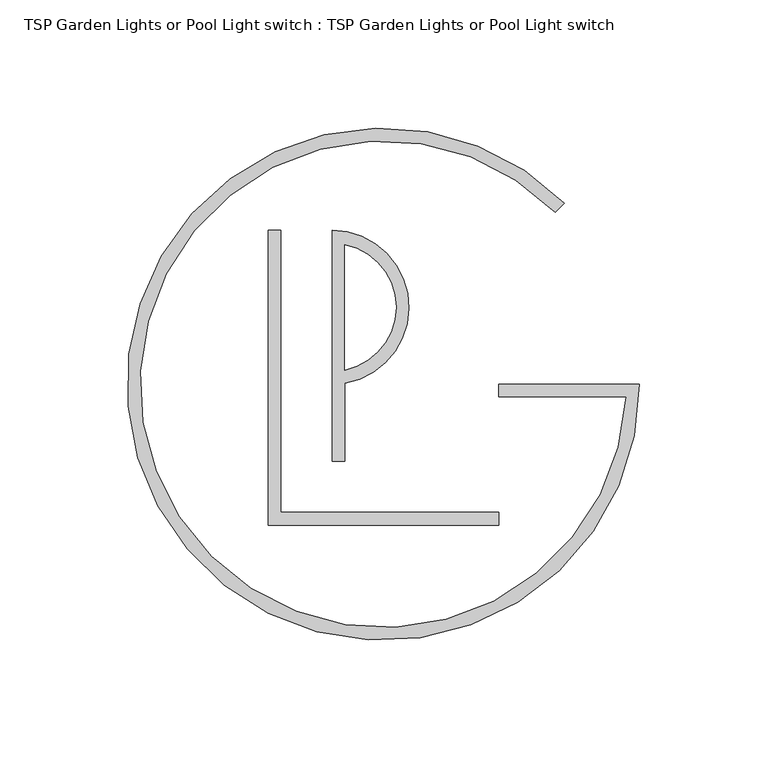
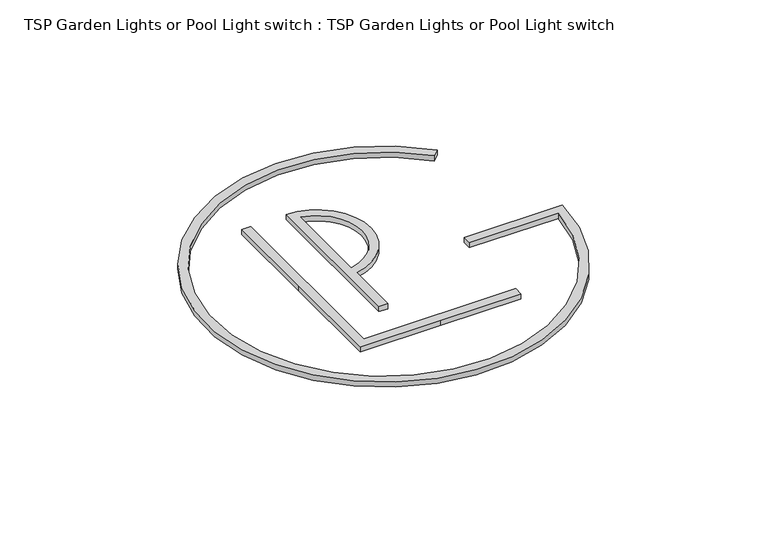
"""IFC4 building model written with IfcOpenShell, lengths in millimetres: proxy geometry, TSP Garden Lights or Pool Light switch : TSP Garden Lights or Pool Light switch."""

from ifc_helpers import new_model, si_unit, point, frame_2d, origin, origin_with_axes, origin_2d, place, context, project, spatial, polyline, circle_curve, trimmed, segment, composite_curve, outline, extrude, source, transform, mapped, element, save


def tsp_garden_lights_or_pool_light_switch_tsp_garden_lights_or_a109b32c(model_context):
    return source(origin(), model_context, "Body", "SweptSolid", [
        extrude(outline(composite_curve([segment(trimmed(circle_curve(origin_2d(), 100.0), [point((100.0, 0.0))], [point((70.7106781, 70.7106781))], False, "CARTESIAN"), True, "CONTINUOUS"), segment(polyline([(70.7106781, 70.7106781), (67.1751442, 67.1751442)]), True, "CONTINUOUS"), segment(trimmed(circle_curve(origin_2d(), 95.0), [point((67.1751442, 67.1751442))], [point((94.8683298, -5.0))], True, "CARTESIAN"), True, "CONTINUOUS"), segment(polyline([(94.8683298, -5.0), (45.0, -5.0), (45.0, 0.0), (100.0, 0.0)]), True, "CONTINUOUS")], self_intersect=False)), origin_with_axes(), (0.0, 0.0, 1.0), 3.0),
        extrude(outline(polyline([(45.0, -55.0), (0.0, -55.0), (-45.0, -55.0), (-45.0, 5.0), (-45.0, 60.0), (-40.0, 60.0), (-40.0, -50.0), (45.0, -50.0), (45.0, -55.0)])), origin_with_axes(), (0.0, 0.0, 1.0), 3.0),
        extrude(outline(composite_curve([segment(polyline([(-20.0, -30.0), (-20.0, 60.0)]), True, "CONTINUOUS"), segment(trimmed(circle_curve(frame_2d((-20.0, 30.0)), 30.0), [point((-20.0, 60.0))], [point((-15.0, 0.4196011))], False, "CARTESIAN"), True, "CONTINUOUS"), segment(polyline([(-15.0, 0.4196011), (-15.0, -30.0), (-20.0, -30.0)]), True, "CONTINUOUS")], self_intersect=False), holes=[composite_curve([segment(polyline([(-15.0, 54.4948974), (-15.0, 5.5051026)]), True, "CONTINUOUS"), segment(trimmed(circle_curve(frame_2d((-20.0, 30.0)), 25.0), [point((-15.0, 5.5051026))], [point((-15.0, 54.4948974))], True, "CARTESIAN"), True, "CONTINUOUS")], self_intersect=False)]), origin_with_axes(), (0.0, 0.0, 1.0), 3.0),
    ])


if __name__ == "__main__":
    model = new_model("IFC4")
    model_context = context("Model", 3, world=origin())
    ifc_project = project(units=[si_unit("LENGTHUNIT", "METRE", prefix="MILLI")], contexts=[model_context])
    site = spatial("IfcSite", under=ifc_project)
    building = spatial("IfcBuilding", under=site)
    placement = place(None, origin())
    tsp_garden_lights_or_pool_light_switch_tsp_garden_lights_or_shape = tsp_garden_lights_or_pool_light_switch_tsp_garden_lights_or_a109b32c(model_context)
    element("IfcBuildingElementProxy", 1, Name="TSP Garden Lights or Pool Light switch : TSP Garden Lights or Pool Light switch", ObjectType="TSP Garden Lights or Pool Light switch : TSP Garden Lights or Pool Light switch", at=placement, inside=building, context=model_context, shape_type="MappedRepresentation", body=[
        mapped(tsp_garden_lights_or_pool_light_switch_tsp_garden_lights_or_shape, transform((0.0, 0.0, 0.0), x_axis=(1.0, 0.0, 0.0), y_axis=(0.0, 1.0, 0.0), z_axis=(0.0, 0.0, 1.0))),
    ])
    save(model, "model.ifc")

# Revit data of these elements
# Type "TSP Garden Lights or Pool Light switch : TSP Garden Lights or Pool Light switch"
#   Model = "TSP_ELEC220GLPL"
#   Default Elevation = 0
# Element 1 (IfcBuildingElementProxy, "TSP Garden Lights or Pool Light switch : TSP Garden Lights or Pool Light switch")
#   Materials on its faces: "Plastic, Opaque Black"
# Materials
#   "Plastic, Opaque Black": class "Plastic", colour RGB 0 0 0, transparency 0.7, Description = "Plastic, generic, opaque black", Cost = 0
